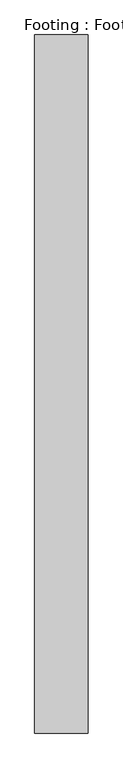
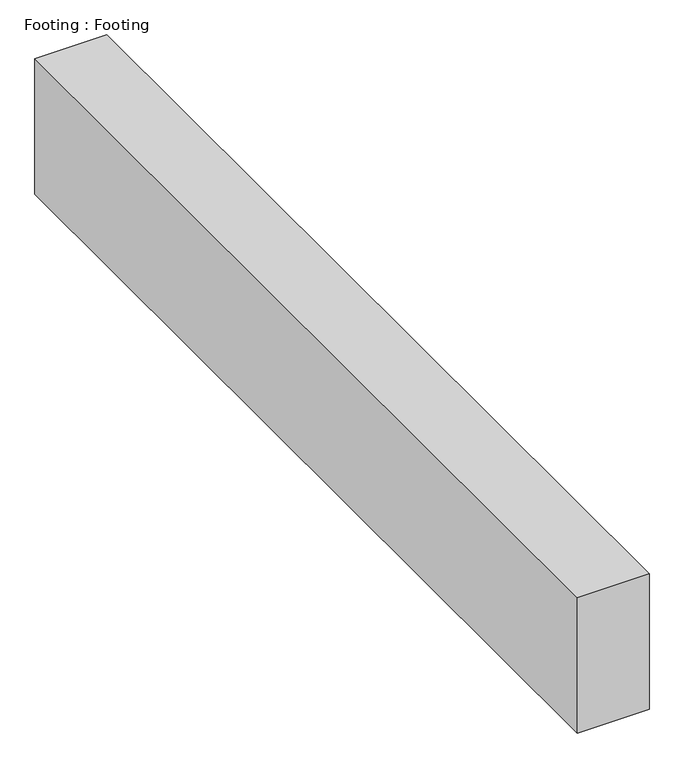
"""IFC4 building model written with IfcOpenShell, lengths in millimetres: proxy geometry, Footing : Footing."""

from ifc_helpers import new_model, si_unit, frame, origin, place, context, project, spatial, polyline, outline, extrude, source, transform, mapped, element, save


def footing_footing_936b6e60(model_context):
    return source(origin(), model_context, "Body", "SweptSolid", [
        extrude(outline(polyline([(-10098.4737014, 7982.1531721), (-10250.8737014, 7982.1531721), (-10250.8737014, 9982.1531721), (-10098.4737014, 9982.1531721), (-10098.4737014, 7982.1531721)])), frame((0.0, 0.0, 32314.8961275), z_axis=(0.0, 0.0, 1.0), x_axis=(1.0, 0.0, 0.0)), (0.0, 0.0, 1.0), 304.8078786),
    ])


if __name__ == "__main__":
    model = new_model("IFC4")
    model_context = context("Model", 3, world=origin())
    ifc_project = project(units=[si_unit("LENGTHUNIT", "METRE", prefix="MILLI")], contexts=[model_context])
    site = spatial("IfcSite", under=ifc_project)
    building = spatial("IfcBuilding", under=site)
    placement = place(None, origin())
    footing_footing_shape = footing_footing_936b6e60(model_context)
    element("IfcBuildingElementProxy", 1, Name="Footing : Footing", ObjectType="Footing : Footing", at=placement, inside=building, context=model_context, shape_type="MappedRepresentation", body=[
        mapped(footing_footing_shape, transform((0.0, 0.0, 0.0), x_axis=(1.0, 0.0, 0.0), y_axis=(0.0, 1.0, 0.0), z_axis=(0.0, 0.0, 1.0))),
    ])
    save(model, "model.ifc")

# Revit data of these elements
# Type "Footing : Footing"
#   NameOverride = "Footing"
# Element 1 (IfcBuildingElementProxy, "Footing : Footing")
#   Materials on its faces: "CONCRETE FOOTING - SEE STRUCTURAL DWGS"
# Materials
#   "CONCRETE FOOTING - SEE STRUCTURAL DWGS": class "Unassigned", colour RGB 128 128 128, transparency 0
